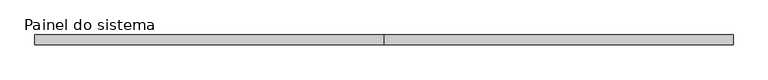
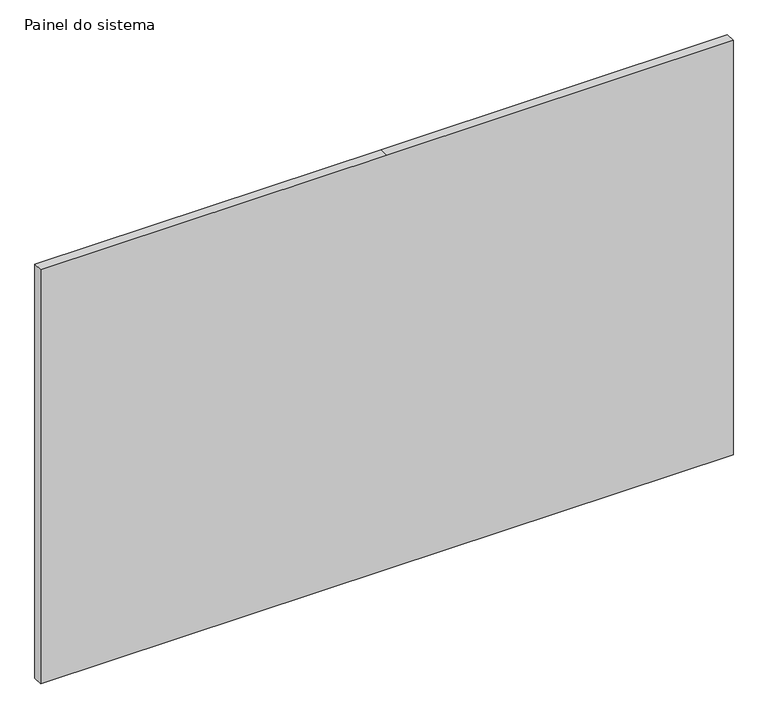
"""IFC4 building model written with IfcOpenShell, lengths in millimetres: plate geometry, Painel do sistema : Envidraçado."""

from ifc_helpers import new_model, si_unit, frame, origin, place, context, project, spatial, polyline, outline, extrude, source, transform, mapped, element, save


def painel_do_sistema_af529942(model_context):
    return source(origin(), model_context, "Body", "SweptSolid", [
        extrude(outline(polyline([(0.0, -890.0), (0.0, 0.0), (0.0, 890.0), (1125.0, 890.0), (1125.0, 0.0), (1125.0, -890.0), (0.0, -890.0)])), frame((0.0, 24.5, 0.0), z_axis=(0.0, 1.0, 0.0), x_axis=(0.0, 0.0, 1.0)), (0.0, 0.0, 1.0), 25.0),
    ])


if __name__ == "__main__":
    model = new_model("IFC4")
    model_context = context("Model", 3, world=origin())
    ifc_project = project(units=[si_unit("LENGTHUNIT", "METRE", prefix="MILLI")], contexts=[model_context])
    site = spatial("IfcSite", under=ifc_project)
    building = spatial("IfcBuilding", under=site)
    placement = place(None, origin())
    painel_do_sistema_shape = painel_do_sistema_af529942(model_context)
    element("IfcPlate", 1, ObjectType="Painel do sistema : Envidraçado", at=placement, inside=building, context=model_context, shape_type="MappedRepresentation", body=[
        mapped(painel_do_sistema_shape, transform((0.0, 0.0, 0.0), x_axis=(1.0, 0.0, 0.0), y_axis=(0.0, 1.0, 0.0), z_axis=(0.0, 0.0, 1.0))),
    ])
    save(model, "model.ifc")

# Revit data of these elements
# Type "Painel do sistema : Envidraçado"
#   Construction Type Id = "GSP4R"
#   Analytic Construction = "Vidraça única Pilkington 1/8 pol"
#   Visual Light Transmittance = 0.9
#   Solar Heat Gain Coefficient = 0.86
#   Heat Transfer Coefficient (U) = 6.7069 W/(m²·K)
# Element 1 (IfcPlate, "Painel do sistema : Envidraçado")
#   Materials on its faces: "Vidro"
# Materials
#   "Vidro": class "Vidro", colour RGB 0 128 192, transparency 0.9, Description = "Vidro de sílica", Cost = 0
